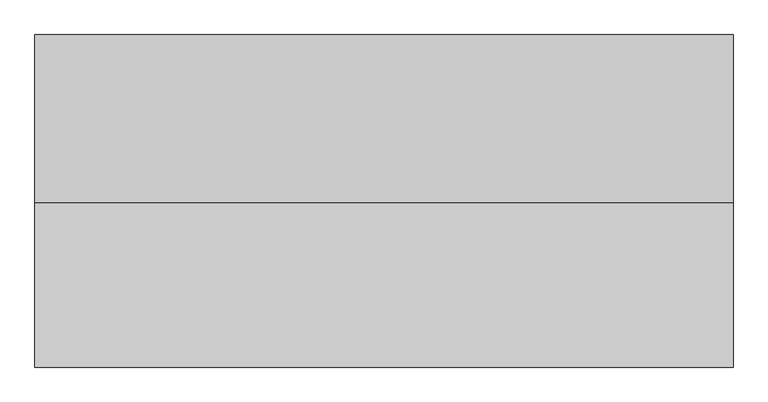
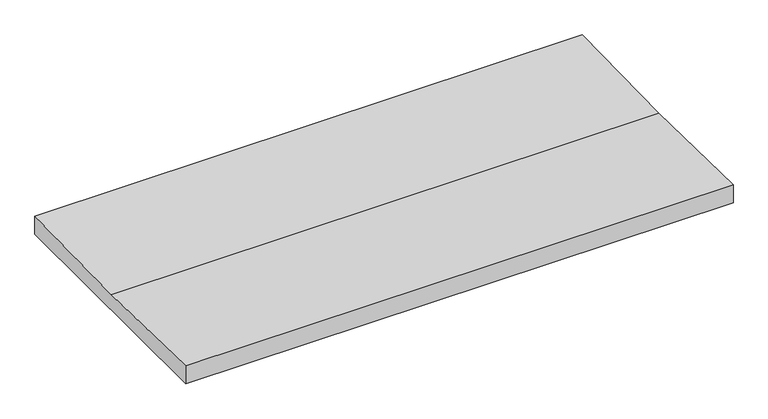
"""IFC4 building model written with IfcOpenShell, lengths in millimetres: proxy geometry, FIRESTONE INSULATION001 : FIRESTONE INSULATION001."""

import ifcopenshell
import ifcopenshell.guid

model = None  # the IFC model being written
_history = None  # IfcOwnerHistory: only IFC2X3 demands one
_inside = {}  # id of a spatial element -> (the spatial element, [elements in it])
_under = {}  # id of a project, library or spatial element -> (it, [spatial elements below it])
_declared = {}  # id of a project -> (the project, [libraries it declares])
_typed = {}  # id of a type object -> (the type object, [elements of that type])
_made_of = {}  # id of a material, layer set ... -> (it, [elements and type objects made of it])


def new_model(schema):
    """Start an empty IFC model of exactly this schema.

    Asked for "IFC4X3", IfcOpenShell would pick the latest addendum, in which some entities
    have other attributes; the version numbers below select the first issue.
    IFC2X3 requires an IfcOwnerHistory on every rooted entity: one is made here for all.
    """
    global model, _history
    if schema == "IFC4X3":
        model = ifcopenshell.file(schema_version=(4, 3, 0, 0))
    else:
        model = ifcopenshell.file(schema=schema)
    _inside.clear()
    _under.clear()
    _declared.clear()
    _typed.clear()
    _made_of.clear()
    _history = None
    if model.schema == "IFC2X3":
        org = make("IfcOrganization", Name="unknown")
        user = make(
            "IfcPersonAndOrganization",
            ThePerson=make("IfcPerson", FamilyName="unknown"),
            TheOrganization=org,
        )
        app = make(
            "IfcApplication",
            ApplicationDeveloper=org,
            Version="unknown",
            ApplicationFullName="unknown",
            ApplicationIdentifier="unknown",
        )
        _history = make(
            "IfcOwnerHistory",
            OwningUser=user,
            OwningApplication=app,
            ChangeAction="ADDED",
            CreationDate=0,
        )
    return model


def make(cls, **values):
    """One entity of the class cls with the attributes given. An attribute that is None is left unset."""
    return model.create_entity(
        cls, **{name: value for name, value in values.items() if value is not None}
    )


def rooted(cls, **values):
    """An entity with a GlobalId (a new one), such as an element, a storey or a relation."""
    return make(cls, GlobalId=ifcopenshell.guid.new(), OwnerHistory=_history, **values)


def si_unit(unit_type, name, prefix=None):
    """IfcSIUnit, for example si_unit("LENGTHUNIT", "METRE", prefix="MILLI")."""
    return make("IfcSIUnit", UnitType=unit_type, Prefix=prefix, Name=name)


def assignment(units):
    """IfcUnitAssignment: the units of a project."""
    return None if units is None else make("IfcUnitAssignment", Units=units)


def point(xyz):
    """IfcCartesianPoint."""
    return None if xyz is None else make("IfcCartesianPoint", Coordinates=xyz)


def direction(xyz):
    """IfcDirection."""
    return None if xyz is None else make("IfcDirection", DirectionRatios=xyz)


def frame(location, z_axis=None, x_axis=None):
    """IfcAxis2Placement3D, a coordinate frame: its origin and axes. An axis left out is left unset."""
    return make(
        "IfcAxis2Placement3D",
        Location=point(location),
        Axis=direction(z_axis),
        RefDirection=direction(x_axis),
    )


def origin():
    """The frame at (0, 0, 0) with its axes left unset."""
    return frame((0.0, 0.0, 0.0))


def place(relative_to, where):
    """IfcLocalPlacement: puts the frame where relative to a parent placement (None: the world)."""
    return make(
        "IfcLocalPlacement", PlacementRelTo=relative_to, RelativePlacement=where
    )


def context(
    kind, dimensions, precision=None, world=None, true_north=None, identifier=None
):
    """IfcGeometricRepresentationContext, for example the 3D "Model" context."""
    return make(
        "IfcGeometricRepresentationContext",
        ContextIdentifier=identifier,
        ContextType=kind,
        CoordinateSpaceDimension=dimensions,
        Precision=precision,
        WorldCoordinateSystem=world,
        TrueNorth=true_north,
    )


def project(units=None, contexts=None):
    """IfcProject with its units and contexts."""
    return rooted(
        "IfcProject",
        Name="project",
        RepresentationContexts=contexts,
        UnitsInContext=assignment(units),
    )


def spatial(cls, under=None, at=None, **own):
    """A site, building, storey or space (cls), placed at a placement, below another one or the project."""
    s = rooted(cls, ObjectPlacement=at, **own)
    if under is not None:
        _under.setdefault(under.id(), (under, []))[1].append(s)
    return s


def polyline(points):
    """IfcPolyline through the points."""
    return make("IfcPolyline", Points=[point(p) for p in points])


def outline(outer, holes=None, kind="AREA"):
    """IfcArbitraryClosedProfileDef: a profile drawn as a closed curve; with holes, ...WithVoids."""
    if holes is None:
        return make("IfcArbitraryClosedProfileDef", ProfileType=kind, OuterCurve=outer)
    return make(
        "IfcArbitraryProfileDefWithVoids",
        ProfileType=kind,
        OuterCurve=outer,
        InnerCurves=holes,
    )


def extrude(swept, where, along, depth):
    """IfcExtrudedAreaSolid: the profile swept, set in the frame where, extruded along a direction by depth."""
    return make(
        "IfcExtrudedAreaSolid",
        SweptArea=swept,
        Position=where,
        ExtrudedDirection=direction(along),
        Depth=depth,
    )


def shape(context_of_items, identifier, shape_type, items):
    """IfcShapeRepresentation: the items that make up one representation, for example the "Body"."""
    return make(
        "IfcShapeRepresentation",
        ContextOfItems=context_of_items,
        RepresentationIdentifier=identifier,
        RepresentationType=shape_type,
        Items=items,
    )


def source(mapping_origin, context_of_items, identifier, shape_type, items):
    """IfcRepresentationMap: a shape defined once, which mapped items show again and again."""
    return make(
        "IfcRepresentationMap",
        MappingOrigin=mapping_origin,
        MappedRepresentation=shape(context_of_items, identifier, shape_type, items),
    )


def transform(
    local_origin,
    x_axis=None,
    y_axis=None,
    z_axis=None,
    scale=None,
    scale2=None,
    scale3=None,
    uniform=True,
):
    """IfcCartesianTransformationOperator3D, or its non-uniform kind. x_axis, y_axis, z_axis: its Axis1, 2, 3."""
    if uniform:
        return make(
            "IfcCartesianTransformationOperator3D",
            Axis1=direction(x_axis),
            Axis2=direction(y_axis),
            LocalOrigin=point(local_origin),
            Scale=scale,
            Axis3=direction(z_axis),
        )
    return make(
        "IfcCartesianTransformationOperator3DnonUniform",
        Axis1=direction(x_axis),
        Axis2=direction(y_axis),
        LocalOrigin=point(local_origin),
        Scale=scale,
        Axis3=direction(z_axis),
        Scale2=scale2,
        Scale3=scale3,
    )


def mapped(mapping_source, mapping_target):
    """IfcMappedItem: shows the shape of a source again, moved by a transform."""
    return make(
        "IfcMappedItem", MappingSource=mapping_source, MappingTarget=mapping_target
    )


def made_of(thing, what):
    """Note that an element or type object is made of a material, layer set ...; save() writes the relation."""
    if what is not None:
        _made_of.setdefault(what.id(), (what, []))[1].append(thing)
    return thing


def element(
    cls,
    number,
    at=None,
    inside=None,
    cuts=None,
    type_object=None,
    material=None,
    context=None,
    identifier="Body",
    shape_type=None,
    held_by="IfcProductDefinitionShape",
    body=None,
    shapes=None,
    **own,
):
    """One element of the class cls, such as IfcWall. Its Tag is "e" and its number.

    at: its placement. inside: the storey or other place that contains it. cuts: it is an
    opening in that element (IfcRelVoidsElement). A single representation is given by context,
    identifier, shape_type and body (its items); several are given by shapes. held_by: the class
    of the entity that holds the representations. save() writes the other relations.
    """
    e = rooted(cls, Tag="e%d" % number, ObjectPlacement=at, **own)
    if body is not None:
        shapes = [shape(context, identifier, shape_type, body)]
    if shapes is not None:
        e.Representation = make(held_by, Representations=shapes)
    if inside is not None:
        _inside.setdefault(inside.id(), (inside, []))[1].append(e)
    if cuts is not None:
        rooted(
            "IfcRelVoidsElement", RelatingBuildingElement=cuts, RelatedOpeningElement=e
        )
    if type_object is not None:
        _typed.setdefault(type_object.id(), (type_object, []))[1].append(e)
    return made_of(e, material)


def aggregate(whole, parts):
    """IfcRelAggregates: a whole, such as a stair, and the parts it consists of."""
    return rooted("IfcRelAggregates", RelatingObject=whole, RelatedObjects=parts)


def save(model, path):
    """Write the relations noted so far, then the file.

    IfcRelAggregates (storeys below a building ...), IfcRelContainedInSpatialStructure (elements
    in a storey), IfcRelDefinesByType, IfcRelAssociatesMaterial and IfcRelDeclares: one each for
    every whole, place, type object, material and project.
    """
    for whole, parts in _under.values():
        aggregate(whole, parts)
    for where, things in _inside.values():
        rooted(
            "IfcRelContainedInSpatialStructure",
            RelatedElements=things,
            RelatingStructure=where,
        )
    for kind, things in _typed.values():
        rooted("IfcRelDefinesByType", RelatedObjects=things, RelatingType=kind)
    for what, things in _made_of.values():
        rooted("IfcRelAssociatesMaterial", RelatedObjects=things, RelatingMaterial=what)
    for by, libraries in _declared.values():
        rooted("IfcRelDeclares", RelatingContext=by, RelatedDefinitions=libraries)
    model.write(path)


def generic_models_233e500c(model_context):
    return source(origin(), model_context, "Body", "SweptSolid", [
        extrude(outline(polyline([(-5343.2581759, 40201.5164062), (-4872.9612169, 40191.7185529), (-4390.315464, 40201.5164062), (-4390.315464, 40131.746), (-5343.2581759, 40131.746), (-5343.2581759, 40201.5164062)])), frame((12382.7678845, 0.0, 0.0), z_axis=(1.0, 0.0, 0.0), x_axis=(0.0, 1.0, 0.0)), (0.0, 0.0, 1.0), 2000.25),
    ])


if __name__ == "__main__":
    model = new_model("IFC4")
    model_context = context("Model", 3, world=origin())
    ifc_project = project(units=[si_unit("LENGTHUNIT", "METRE", prefix="MILLI")], contexts=[model_context])
    site = spatial("IfcSite", under=ifc_project)
    building = spatial("IfcBuilding", under=site)
    placement = place(None, origin())
    generic_models_shape = generic_models_233e500c(model_context)
    element("IfcBuildingElementProxy", 1, Name="FIRESTONE INSULATION001 : FIRESTONE INSULATION001", ObjectType="FIRESTONE INSULATION001 : FIRESTONE INSULATION001", at=placement, inside=building, context=model_context, shape_type="MappedRepresentation", body=[
        mapped(generic_models_shape, transform((0.0, 0.0, 0.0), x_axis=(1.0, 0.0, 0.0), y_axis=(0.0, 1.0, 0.0), z_axis=(0.0, 0.0, 1.0))),
    ])
    save(model, "model.ifc")

# Revit data of these elements
# Type "FIRESTONE INSULATION001 : FIRESTONE INSULATION001"
#   NameOverride = "FIRESTONE INSULATION001"
# Element 1 (IfcBuildingElementProxy, "FIRESTONE INSULATION001 : FIRESTONE INSULATION001")
#   Materials on its faces: "TAPERED 2X SLEEPERS - SLOPED TO DRAIN"
# Materials
#   "TAPERED 2X SLEEPERS - SLOPED TO DRAIN": class "Unassigned", colour RGB 234 198 178, transparency 0
